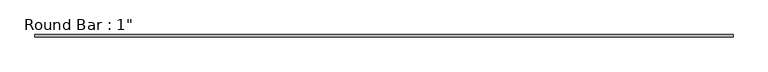
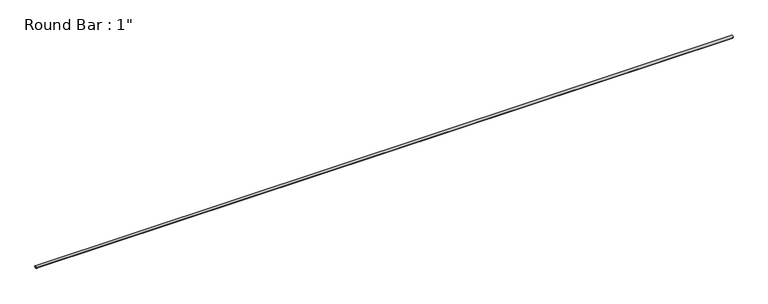
"""IFC4 building model written with IfcOpenShell, lengths in millimetres: member geometry."""

from ifc_helpers import new_model, si_unit, point, frame, origin, origin_2d, place, context, project, spatial, circle_curve, trimmed, segment, composite_curve, outline, extrude, source, transform, mapped, element, save


def member_357c6e14(model_context):
    return source(origin(), model_context, "Body", "SweptSolid", [
        extrude(outline(composite_curve([segment(trimmed(circle_curve(origin_2d(), 12.7), [point((12.7, 0.0))], [point((-12.7, 0.0))], False, "CARTESIAN"), True, "CONTINUOUS"), segment(trimmed(circle_curve(origin_2d(), 12.7), [point((-12.7, 0.0))], [point((12.7, 0.0))], False, "CARTESIAN"), True, "CONTINUOUS")], self_intersect=False)), frame((-3554.2056387, 0.0, 0.0), z_axis=(1.0, 0.0, 0.0), x_axis=(0.0, 1.0, 0.0)), (0.0, 0.0, 1.0), 7108.4112774),
    ])


if __name__ == "__main__":
    model = new_model("IFC4")
    model_context = context("Model", 3, world=origin())
    ifc_project = project(units=[si_unit("LENGTHUNIT", "METRE", prefix="MILLI")], contexts=[model_context])
    site = spatial("IfcSite", under=ifc_project)
    building = spatial("IfcBuilding", under=site)
    placement = place(None, origin())
    member_shape = member_357c6e14(model_context)
    element("IfcMember", 1, ObjectType="Round Bar : 1\"", at=placement, inside=building, context=model_context, shape_type="MappedRepresentation", body=[
        mapped(member_shape, transform((0.0, 0.0, 0.0), x_axis=(1.0, 0.0, 0.0), y_axis=(0.0, 1.0, 0.0), z_axis=(0.0, 0.0, 1.0))),
    ])
    save(model, "model.ifc")

# Revit data of these elements
# Type "Round Bar : 1\""
#   Assembly Code = "B10"
#   W = 0
#   Start Extension Calculation [instance default] = 10' - 0"
#   Start Extension [instance default] = -0' - 0 1/2"
#   End Extension Calculation [instance default] = 10' - 0"
#   End Extension [instance default] = -0' - 0 1/2"
#   Length [instance default] = 5' - 0"
#   d = 0' - 1"
#   A = 0 SF
#   Structural Material [instance default] = Metal - Steel - ASTM A36
# Element 1 (IfcMember, "Round Bar : 1\"")
#   Materials on its faces: "Metal - Steel - ASTM A36"
# Materials
#   "Metal - Steel - ASTM A36": class "Metal", colour RGB 199 199 199, transparency 0
